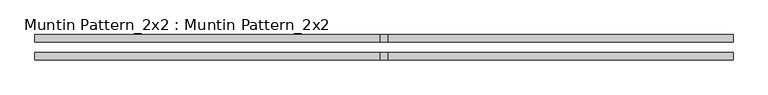
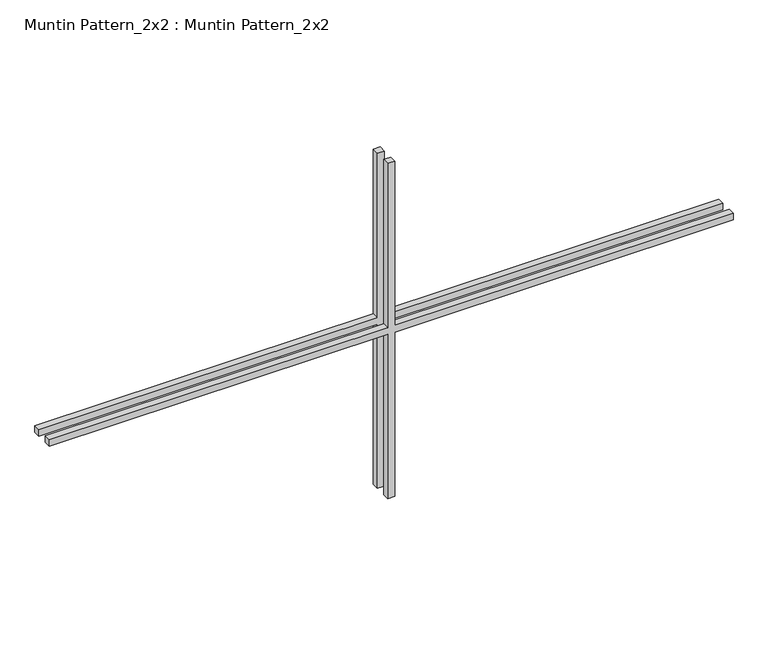
"""IFC4 building model written with IfcOpenShell, lengths in millimetres: proxy geometry, Muntin Pattern_2x2 : Muntin Pattern_2x2."""

from ifc_helpers import new_model, si_unit, frame, origin, place, context, project, spatial, polyline, outline, extrude, source, transform, mapped, element, save


def muntin_pattern_2x2_muntin_pattern_2x2_7f11c842(model_context):
    return source(origin(), model_context, "Body", "SweptSolid", [
        extrude(outline(polyline([(325.4375, -6.35), (325.4375, -615.95), (312.7375, -615.95), (312.7375, -6.35), (0.0, -6.35), (0.0, 6.35), (312.7375, 6.35), (312.7375, 615.95), (325.4375, 615.95), (325.4375, 6.35), (638.175, 6.35), (638.175, -6.35), (325.4375, -6.35)])), frame((0.0, 9.525, 0.0), z_axis=(0.0, 1.0, 0.0), x_axis=(0.0, 0.0, 1.0)), (0.0, 0.0, 1.0), 12.7),
        extrude(outline(polyline([(325.4375, -6.35), (325.4375, -615.95), (312.7375, -615.95), (312.7375, -6.35), (0.0, -6.35), (0.0, 6.35), (312.7375, 6.35), (312.7375, 615.95), (325.4375, 615.95), (325.4375, 6.35), (638.175, 6.35), (638.175, -6.35), (325.4375, -6.35)])), frame((0.0, -22.225, 0.0), z_axis=(0.0, 1.0, 0.0), x_axis=(0.0, 0.0, 1.0)), (0.0, 0.0, 1.0), 12.7),
    ])


if __name__ == "__main__":
    model = new_model("IFC4")
    model_context = context("Model", 3, world=origin())
    ifc_project = project(units=[si_unit("LENGTHUNIT", "METRE", prefix="MILLI")], contexts=[model_context])
    site = spatial("IfcSite", under=ifc_project)
    building = spatial("IfcBuilding", under=site)
    placement = place(None, origin())
    muntin_pattern_2x2_muntin_pattern_2x2_shape = muntin_pattern_2x2_muntin_pattern_2x2_7f11c842(model_context)
    element("IfcBuildingElementProxy", 1, Name="Muntin Pattern_2x2 : Muntin Pattern_2x2", ObjectType="Muntin Pattern_2x2 : Muntin Pattern_2x2", at=placement, inside=building, context=model_context, shape_type="MappedRepresentation", body=[
        mapped(muntin_pattern_2x2_muntin_pattern_2x2_shape, transform((0.0, 0.0, 0.0), x_axis=(1.0, 0.0, 0.0), y_axis=(0.0, 1.0, 0.0), z_axis=(0.0, 0.0, 1.0))),
    ])
    save(model, "model.ifc")

# Revit data of these elements
# Type "Muntin Pattern_2x2 : Muntin Pattern_2x2"
#   Width [instance default] = 4' - 0"
#   Thickness = 0' - 0 1/2"
#   Height [instance default] = 4' - 0"
#   Distance = 0' - 0 3/4"
#   Interior Material [instance default] = none
#   Exterior Material [instance default] = none
# Element 1 (IfcBuildingElementProxy, "Muntin Pattern_2x2 : Muntin Pattern_2x2")
#   Width = 4' - 0 1/2"
#   Height = 2' - 1 1/8"
#   Interior Material = Wood - Stained
#   Exterior Material = Clad - White
#   Materials on its faces: "Clad - White", "Wood - Stained"
# Materials
#   "Clad - White": class "Wood", colour RGB 242 242 238, transparency 0, Cost = 0
#   "Wood - Stained": class "Wood", colour RGB 224 178 126, transparency 0, Cost = 0
